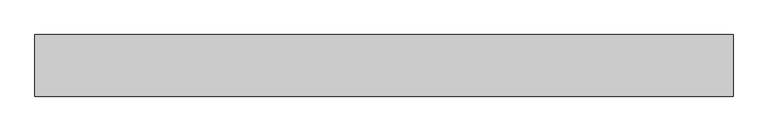
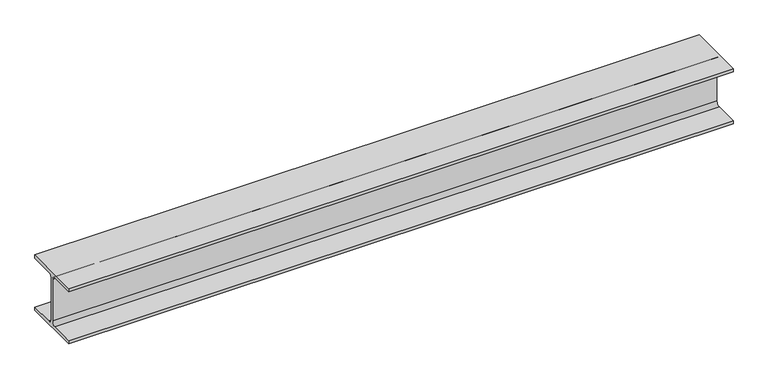
"""IFC4 building model written with IfcOpenShell, lengths in millimetres: beam geometry, 0912_Steel Framing_H-KSD3502 : H_SB_ASB_H-200x200x8x12."""

from ifc_helpers import new_model, si_unit, point, frame, frame_2d, origin, place, context, project, spatial, polyline, circle_curve, trimmed, segment, composite_curve, outline, extrude, source, transform, mapped, element, save


def beam_613f7d83(model_context):
    return source(origin(), model_context, "Body", "SweptSolid", [
        extrude(outline(composite_curve([segment(polyline([(100.0, -88.0), (100.0, -100.0), (-100.0, -100.0), (-100.0, -88.0), (-17.0, -88.0)]), True, "CONTINUOUS"), segment(trimmed(circle_curve(frame_2d((-17.0, -75.0)), 13.0), [point((-17.0, -88.0))], [point((-4.0, -75.0))], True, "CARTESIAN"), True, "CONTINUOUS"), segment(polyline([(-4.0, -75.0), (-4.0, 75.0)]), True, "CONTINUOUS"), segment(trimmed(circle_curve(frame_2d((-17.0, 75.0)), 13.0), [point((-4.0, 75.0))], [point((-17.0, 88.0))], True, "CARTESIAN"), True, "CONTINUOUS"), segment(polyline([(-17.0, 88.0), (-100.0, 88.0), (-100.0, 100.0), (100.0, 100.0), (100.0, 88.0), (17.0, 88.0)]), True, "CONTINUOUS"), segment(trimmed(circle_curve(frame_2d((17.0, 75.0)), 13.0), [point((17.0, 88.0))], [point((4.0, 75.0))], True, "CARTESIAN"), True, "CONTINUOUS"), segment(polyline([(4.0, 75.0), (4.0, -75.0)]), True, "CONTINUOUS"), segment(trimmed(circle_curve(frame_2d((17.0, -75.0)), 13.0), [point((4.0, -75.0))], [point((17.0, -88.0))], True, "CARTESIAN"), True, "CONTINUOUS"), segment(polyline([(17.0, -88.0), (100.0, -88.0)]), True, "CONTINUOUS")], self_intersect=False)), frame((-1290.1039273, 0.0, 0.0), z_axis=(1.0, 0.0, 0.0), x_axis=(0.0, 1.0, 0.0)), (0.0, 0.0, 1.0), 2266.3439099),
    ])


if __name__ == "__main__":
    model = new_model("IFC4")
    model_context = context("Model", 3, world=origin())
    ifc_project = project(units=[si_unit("LENGTHUNIT", "METRE", prefix="MILLI")], contexts=[model_context])
    site = spatial("IfcSite", under=ifc_project)
    building = spatial("IfcBuilding", under=site)
    placement = place(None, origin())
    beam_shape = beam_613f7d83(model_context)
    element("IfcBeam", 1, ObjectType="0912_Steel Framing_H-KSD3502 : H_SB_ASB_H-200x200x8x12", at=placement, inside=building, context=model_context, shape_type="MappedRepresentation", body=[
        mapped(beam_shape, transform((0.0, 0.0, 0.0), x_axis=(1.0, 0.0, 0.0), y_axis=(0.0, 1.0, 0.0), z_axis=(0.0, 0.0, 1.0))),
    ])
    save(model, "model.ifc")

# Revit data of these elements
# Type "0912_Steel Framing_H-KSD3502 : H_SB_ASB_H-200x200x8x12"
#   H_WM Code_1 = "S01AA002-00001 | Main Steel Structure Fabrication Work | Shelter/Building | Medium Steel - Standard (90KG/M>Weight≥30KG/M) | Material: (   )"
#   H_WM Code_2 = "S03AA028-00001 | Main Steel Structure Erection Work | Shelter/Building | Medium Steel (90KG/M>Weight≥30KG/M) | Material: (   )"
#   H_WM Code_3 = "S01AA010-00001 | Main Steel Structure Fabrication Work | Shelter/Building | Steel Painting/Coating | for Non-Fireproofed Steel Surface, Surface Preparation, Primer, Second & Final Coat | Material: (   )"
#   H_Q'ty Cal Type Tag = "SB-Q2"
#   Width = 20.0 cm
#   Web Thickness = 0.8 cm
#   Web Fillet = 1.3 cm
#   Warping Constant = 141000.0 cm⁶
#   W = 0
#   Torsional Moment of Inertia = 26.2485 cm⁴
#   Section Area = 63.53 cm²
#   Plastic Modulus weak axis = 244.0 cm³
#   Plastic Modulus strong axis = 525.0 cm³
#   Perimeter = 1.16 m²/m
#   Nominal Weight = 49.90 kgf/m
#   Moment of Inertia weak axis = 1600.00 cm⁴
#   Moment of Inertia strong axis = 4720.00 cm⁴
#   Height = 20.0 cm
#   Flange Thickness = 1.2 cm
#   Elastic Modulus weak axis = 160.0 cm³
#   Elastic Modulus strong axis = 472.0 cm³
#   Centroid Vertical = 10.0 cm
#   Centroid Horizontal = 10.0 cm
#   Ix = 47200000
#   Length [instance default] = 1.5240 m
#   Zx = 525000
#   b = 0.2000 m
#   h = 0.2000 m
#   r = 0.0130 m
#   s = 0.0080 m
#   t = 0.0120 m
#   A = 0.006353 m²
#   Structural Material [instance default] = Steel, 45-345
#   Assembly Code = ""
# Element 1 (IfcBeam, "0912_Steel Framing_H-KSD3502 : H_SB_ASB_H-200x200x8x12")
#   Structural Material = none
# Materials
#   "Steel, 45-345": class "Metal", colour RGB 189 187 185, transparency 0, Description = "Steel 345 MPa", Cost = 0
